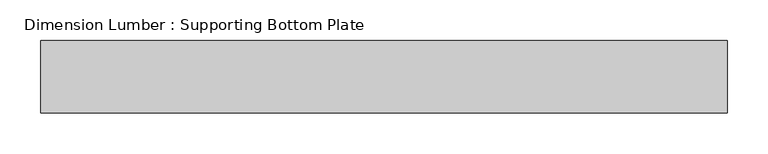
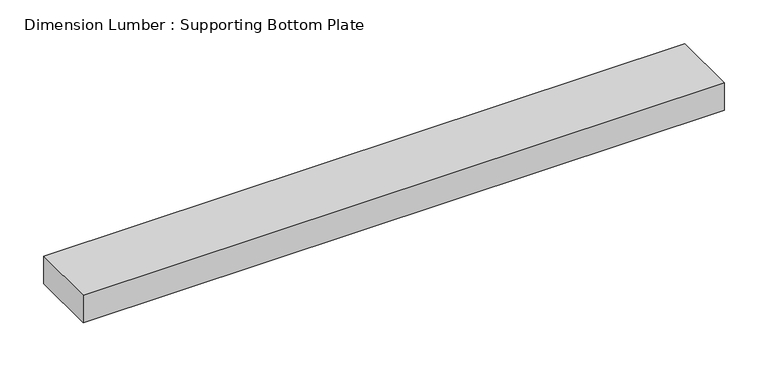
"""IFC4 building model written with IfcOpenShell, lengths in millimetres: beam geometry, Dimension Lumber : Supporting Bottom Plate."""

from ifc_helpers import new_model, si_unit, frame, origin, place, context, project, spatial, polyline, outline, extrude, source, transform, mapped, element, save


def dimension_lumber_supporting_bottom_plate_d3939b75(model_context):
    return source(origin(), model_context, "Body", "SweptSolid", [
        extrude(outline(polyline([(398.375, 44.45), (398.375, -44.45), (-442.825, -44.45), (-442.825, 44.45), (398.375, 44.45)])), frame((0.0, 0.0, -19.05), z_axis=(0.0, 0.0, 1.0), x_axis=(1.0, 0.0, 0.0)), (0.0, 0.0, 1.0), 38.1),
    ])


if __name__ == "__main__":
    model = new_model("IFC4")
    model_context = context("Model", 3, world=origin())
    ifc_project = project(units=[si_unit("LENGTHUNIT", "METRE", prefix="MILLI")], contexts=[model_context])
    site = spatial("IfcSite", under=ifc_project)
    building = spatial("IfcBuilding", under=site)
    placement = place(None, origin())
    dimension_lumber_supporting_bottom_plate_shape = dimension_lumber_supporting_bottom_plate_d3939b75(model_context)
    element("IfcBeam", 1, ObjectType="Dimension Lumber : Supporting Bottom Plate", at=placement, inside=building, context=model_context, shape_type="MappedRepresentation", body=[
        mapped(dimension_lumber_supporting_bottom_plate_shape, transform((0.0, 0.0, 0.0), x_axis=(1.0, 0.0, 0.0), y_axis=(0.0, 1.0, 0.0), z_axis=(0.0, 0.0, 1.0))),
    ])
    save(model, "model.ifc")

# Revit data of these elements
# Type "Dimension Lumber : Supporting Bottom Plate"
#   Assembly Code = "B10"
#   A = 0.0364583 SF
#   Length [instance default] = 5' - 0"
#   b = 0' - 3 1/2"
#   d = 0' - 1 1/2"
#   Structural Material [instance default] = Softwood, Lumber
# Element 1 (IfcBeam, "Dimension Lumber : Supporting Bottom Plate")
#   Structural Material = Douglas Fir #2
#   Materials on its faces: "Douglas Fir #2"
# Materials
#   "Softwood, Lumber": class "Wood", colour RGB 223 192 134, transparency 0, Description = "Pinus Echinata", Cost = 0
#   "Douglas Fir #2": class "Wood", colour RGB 223 192 134, transparency 0, Description = "Pinus Echinata", Cost = 0
